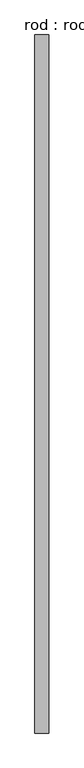
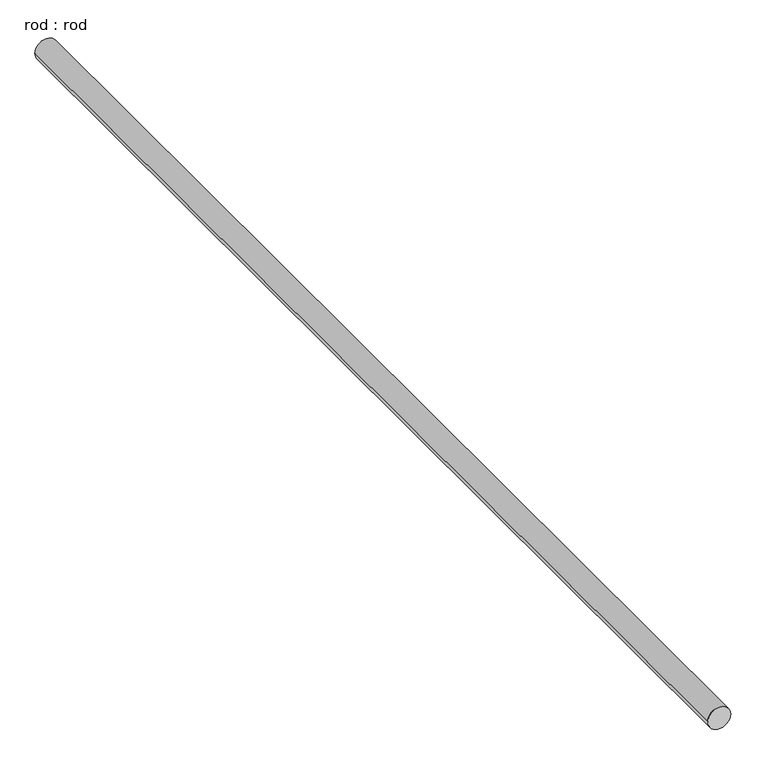
"""IFC4 building model written with IfcOpenShell, lengths in millimetres: proxy geometry, rod : rod."""

import ifcopenshell
import ifcopenshell.guid

model = None  # the IFC model being written
_history = None  # IfcOwnerHistory: only IFC2X3 demands one
_inside = {}  # id of a spatial element -> (the spatial element, [elements in it])
_under = {}  # id of a project, library or spatial element -> (it, [spatial elements below it])
_declared = {}  # id of a project -> (the project, [libraries it declares])
_typed = {}  # id of a type object -> (the type object, [elements of that type])
_made_of = {}  # id of a material, layer set ... -> (it, [elements and type objects made of it])


def new_model(schema):
    """Start an empty IFC model of exactly this schema.

    Asked for "IFC4X3", IfcOpenShell would pick the latest addendum, in which some entities
    have other attributes; the version numbers below select the first issue.
    IFC2X3 requires an IfcOwnerHistory on every rooted entity: one is made here for all.
    """
    global model, _history
    if schema == "IFC4X3":
        model = ifcopenshell.file(schema_version=(4, 3, 0, 0))
    else:
        model = ifcopenshell.file(schema=schema)
    _inside.clear()
    _under.clear()
    _declared.clear()
    _typed.clear()
    _made_of.clear()
    _history = None
    if model.schema == "IFC2X3":
        org = make("IfcOrganization", Name="unknown")
        user = make(
            "IfcPersonAndOrganization",
            ThePerson=make("IfcPerson", FamilyName="unknown"),
            TheOrganization=org,
        )
        app = make(
            "IfcApplication",
            ApplicationDeveloper=org,
            Version="unknown",
            ApplicationFullName="unknown",
            ApplicationIdentifier="unknown",
        )
        _history = make(
            "IfcOwnerHistory",
            OwningUser=user,
            OwningApplication=app,
            ChangeAction="ADDED",
            CreationDate=0,
        )
    return model


def make(cls, **values):
    """One entity of the class cls with the attributes given. An attribute that is None is left unset."""
    return model.create_entity(
        cls, **{name: value for name, value in values.items() if value is not None}
    )


def rooted(cls, **values):
    """An entity with a GlobalId (a new one), such as an element, a storey or a relation."""
    return make(cls, GlobalId=ifcopenshell.guid.new(), OwnerHistory=_history, **values)


def si_unit(unit_type, name, prefix=None):
    """IfcSIUnit, for example si_unit("LENGTHUNIT", "METRE", prefix="MILLI")."""
    return make("IfcSIUnit", UnitType=unit_type, Prefix=prefix, Name=name)


def assignment(units):
    """IfcUnitAssignment: the units of a project."""
    return None if units is None else make("IfcUnitAssignment", Units=units)


def point(xyz):
    """IfcCartesianPoint."""
    return None if xyz is None else make("IfcCartesianPoint", Coordinates=xyz)


def direction(xyz):
    """IfcDirection."""
    return None if xyz is None else make("IfcDirection", DirectionRatios=xyz)


def frame(location, z_axis=None, x_axis=None):
    """IfcAxis2Placement3D, a coordinate frame: its origin and axes. An axis left out is left unset."""
    return make(
        "IfcAxis2Placement3D",
        Location=point(location),
        Axis=direction(z_axis),
        RefDirection=direction(x_axis),
    )


def frame_2d(location, x_axis=None):
    """IfcAxis2Placement2D, a coordinate frame in the plane: its origin and x axis."""
    return make(
        "IfcAxis2Placement2D", Location=point(location), RefDirection=direction(x_axis)
    )


def origin():
    """The frame at (0, 0, 0) with its axes left unset."""
    return frame((0.0, 0.0, 0.0))


def place(relative_to, where):
    """IfcLocalPlacement: puts the frame where relative to a parent placement (None: the world)."""
    return make(
        "IfcLocalPlacement", PlacementRelTo=relative_to, RelativePlacement=where
    )


def context(
    kind, dimensions, precision=None, world=None, true_north=None, identifier=None
):
    """IfcGeometricRepresentationContext, for example the 3D "Model" context."""
    return make(
        "IfcGeometricRepresentationContext",
        ContextIdentifier=identifier,
        ContextType=kind,
        CoordinateSpaceDimension=dimensions,
        Precision=precision,
        WorldCoordinateSystem=world,
        TrueNorth=true_north,
    )


def project(units=None, contexts=None):
    """IfcProject with its units and contexts."""
    return rooted(
        "IfcProject",
        Name="project",
        RepresentationContexts=contexts,
        UnitsInContext=assignment(units),
    )


def spatial(cls, under=None, at=None, **own):
    """A site, building, storey or space (cls), placed at a placement, below another one or the project."""
    s = rooted(cls, ObjectPlacement=at, **own)
    if under is not None:
        _under.setdefault(under.id(), (under, []))[1].append(s)
    return s


def circle_curve(where, radius):
    """IfcCircle in the frame where."""
    return make("IfcCircle", Position=where, Radius=radius)


def trimmed(basis, trim1, trim2, sense, master):
    """IfcTrimmedCurve: the piece of a basis curve between two trims."""
    return make(
        "IfcTrimmedCurve",
        BasisCurve=basis,
        Trim1=trim1,
        Trim2=trim2,
        SenseAgreement=sense,
        MasterRepresentation=master,
    )


def segment(curve, same_sense, transition):
    """IfcCompositeCurveSegment."""
    return make(
        "IfcCompositeCurveSegment",
        Transition=transition,
        SameSense=same_sense,
        ParentCurve=curve,
    )


def composite_curve(segments, self_intersect=None):
    """IfcCompositeCurve: segments joined end to end."""
    return make("IfcCompositeCurve", Segments=segments, SelfIntersect=self_intersect)


def outline(outer, holes=None, kind="AREA"):
    """IfcArbitraryClosedProfileDef: a profile drawn as a closed curve; with holes, ...WithVoids."""
    if holes is None:
        return make("IfcArbitraryClosedProfileDef", ProfileType=kind, OuterCurve=outer)
    return make(
        "IfcArbitraryProfileDefWithVoids",
        ProfileType=kind,
        OuterCurve=outer,
        InnerCurves=holes,
    )


def extrude(swept, where, along, depth):
    """IfcExtrudedAreaSolid: the profile swept, set in the frame where, extruded along a direction by depth."""
    return make(
        "IfcExtrudedAreaSolid",
        SweptArea=swept,
        Position=where,
        ExtrudedDirection=direction(along),
        Depth=depth,
    )


def shape(context_of_items, identifier, shape_type, items):
    """IfcShapeRepresentation: the items that make up one representation, for example the "Body"."""
    return make(
        "IfcShapeRepresentation",
        ContextOfItems=context_of_items,
        RepresentationIdentifier=identifier,
        RepresentationType=shape_type,
        Items=items,
    )


def source(mapping_origin, context_of_items, identifier, shape_type, items):
    """IfcRepresentationMap: a shape defined once, which mapped items show again and again."""
    return make(
        "IfcRepresentationMap",
        MappingOrigin=mapping_origin,
        MappedRepresentation=shape(context_of_items, identifier, shape_type, items),
    )


def transform(
    local_origin,
    x_axis=None,
    y_axis=None,
    z_axis=None,
    scale=None,
    scale2=None,
    scale3=None,
    uniform=True,
):
    """IfcCartesianTransformationOperator3D, or its non-uniform kind. x_axis, y_axis, z_axis: its Axis1, 2, 3."""
    if uniform:
        return make(
            "IfcCartesianTransformationOperator3D",
            Axis1=direction(x_axis),
            Axis2=direction(y_axis),
            LocalOrigin=point(local_origin),
            Scale=scale,
            Axis3=direction(z_axis),
        )
    return make(
        "IfcCartesianTransformationOperator3DnonUniform",
        Axis1=direction(x_axis),
        Axis2=direction(y_axis),
        LocalOrigin=point(local_origin),
        Scale=scale,
        Axis3=direction(z_axis),
        Scale2=scale2,
        Scale3=scale3,
    )


def mapped(mapping_source, mapping_target):
    """IfcMappedItem: shows the shape of a source again, moved by a transform."""
    return make(
        "IfcMappedItem", MappingSource=mapping_source, MappingTarget=mapping_target
    )


def made_of(thing, what):
    """Note that an element or type object is made of a material, layer set ...; save() writes the relation."""
    if what is not None:
        _made_of.setdefault(what.id(), (what, []))[1].append(thing)
    return thing


def element(
    cls,
    number,
    at=None,
    inside=None,
    cuts=None,
    type_object=None,
    material=None,
    context=None,
    identifier="Body",
    shape_type=None,
    held_by="IfcProductDefinitionShape",
    body=None,
    shapes=None,
    **own,
):
    """One element of the class cls, such as IfcWall. Its Tag is "e" and its number.

    at: its placement. inside: the storey or other place that contains it. cuts: it is an
    opening in that element (IfcRelVoidsElement). A single representation is given by context,
    identifier, shape_type and body (its items); several are given by shapes. held_by: the class
    of the entity that holds the representations. save() writes the other relations.
    """
    e = rooted(cls, Tag="e%d" % number, ObjectPlacement=at, **own)
    if body is not None:
        shapes = [shape(context, identifier, shape_type, body)]
    if shapes is not None:
        e.Representation = make(held_by, Representations=shapes)
    if inside is not None:
        _inside.setdefault(inside.id(), (inside, []))[1].append(e)
    if cuts is not None:
        rooted(
            "IfcRelVoidsElement", RelatingBuildingElement=cuts, RelatedOpeningElement=e
        )
    if type_object is not None:
        _typed.setdefault(type_object.id(), (type_object, []))[1].append(e)
    return made_of(e, material)


def aggregate(whole, parts):
    """IfcRelAggregates: a whole, such as a stair, and the parts it consists of."""
    return rooted("IfcRelAggregates", RelatingObject=whole, RelatedObjects=parts)


def save(model, path):
    """Write the relations noted so far, then the file.

    IfcRelAggregates (storeys below a building ...), IfcRelContainedInSpatialStructure (elements
    in a storey), IfcRelDefinesByType, IfcRelAssociatesMaterial and IfcRelDeclares: one each for
    every whole, place, type object, material and project.
    """
    for whole, parts in _under.values():
        aggregate(whole, parts)
    for where, things in _inside.values():
        rooted(
            "IfcRelContainedInSpatialStructure",
            RelatedElements=things,
            RelatingStructure=where,
        )
    for kind, things in _typed.values():
        rooted("IfcRelDefinesByType", RelatedObjects=things, RelatingType=kind)
    for what, things in _made_of.values():
        rooted("IfcRelAssociatesMaterial", RelatedObjects=things, RelatingMaterial=what)
    for by, libraries in _declared.values():
        rooted("IfcRelDeclares", RelatingContext=by, RelatedDefinitions=libraries)
    model.write(path)


def rod_rod_449a3736(model_context):
    return source(origin(), model_context, "Body", "SweptSolid", [
        extrude(outline(composite_curve([segment(trimmed(circle_curve(frame_2d((0.0108462, 0.0)), 200.0), [point((0.0108462, 200.0))], [point((0.0108462, -200.0))], False, "CARTESIAN"), True, "CONTINUOUS"), segment(trimmed(circle_curve(frame_2d((0.0108462, 0.0)), 200.0), [point((0.0108462, -200.0))], [point((0.0108462, 200.0))], False, "CARTESIAN"), True, "CONTINUOUS")], self_intersect=False)), frame((0.0, -6072.4499561, 0.0), z_axis=(0.0, 1.0, 0.0), x_axis=(0.0, 0.0, 1.0)), (0.0, 0.0, 1.0), 20330.3571429),
    ])


if __name__ == "__main__":
    model = new_model("IFC4")
    model_context = context("Model", 3, world=origin())
    ifc_project = project(units=[si_unit("LENGTHUNIT", "METRE", prefix="MILLI")], contexts=[model_context])
    site = spatial("IfcSite", under=ifc_project)
    building = spatial("IfcBuilding", under=site)
    placement = place(None, origin())
    rod_rod_shape = rod_rod_449a3736(model_context)
    element("IfcBuildingElementProxy", 1, Name="rod : rod", ObjectType="rod : rod", at=placement, inside=building, context=model_context, shape_type="MappedRepresentation", body=[
        mapped(rod_rod_shape, transform((0.0, 0.0, 0.0), x_axis=(1.0, 0.0, 0.0), y_axis=(0.0, 1.0, 0.0), z_axis=(0.0, 0.0, 1.0))),
    ])
    save(model, "model.ifc")

# Revit data of these elements
# Type "rod : rod"
#   Default Elevation = 0
